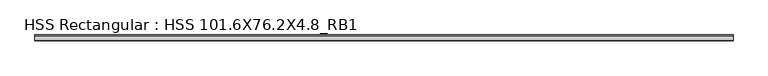
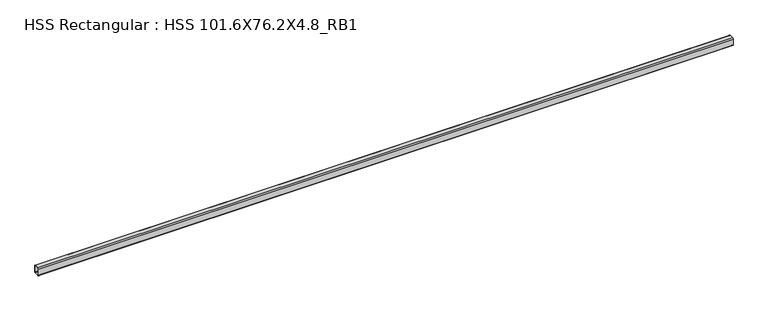
"""IFC4 building model written with IfcOpenShell, lengths in millimetres: beam geometry, HSS Rectangular : HSS 101.6X76.2X4.8_RB1."""

from ifc_helpers import new_model, si_unit, point, frame, frame_2d, origin, place, context, project, spatial, polyline, circle_curve, trimmed, segment, composite_curve, outline, extrude, source, transform, mapped, element, save


def hss_rectangular_hss_101_6x76_2x4_8_rb1_fc7daad9(model_context):
    return source(origin(), model_context, "Body", "SweptSolid", [
        extrude(outline(composite_curve([segment(polyline([(38.1, 41.275), (38.1, -41.275)]), True, "CONTINUOUS"), segment(trimmed(circle_curve(frame_2d((28.575, -41.275)), 9.525), [point((38.1, -41.275))], [point((28.575, -50.8))], False, "CARTESIAN"), True, "CONTINUOUS"), segment(polyline([(28.575, -50.8), (-28.575, -50.8)]), True, "CONTINUOUS"), segment(trimmed(circle_curve(frame_2d((-28.575, -41.275)), 9.525), [point((-28.575, -50.8))], [point((-38.1, -41.275))], False, "CARTESIAN"), True, "CONTINUOUS"), segment(polyline([(-38.1, -41.275), (-38.1, 41.275)]), True, "CONTINUOUS"), segment(trimmed(circle_curve(frame_2d((-28.575, 41.275)), 9.525), [point((-38.1, 41.275))], [point((-28.575, 50.8))], False, "CARTESIAN"), True, "CONTINUOUS"), segment(polyline([(-28.575, 50.8), (28.575, 50.8)]), True, "CONTINUOUS"), segment(trimmed(circle_curve(frame_2d((28.575, 41.275)), 9.525), [point((28.575, 50.8))], [point((38.1, 41.275))], False, "CARTESIAN"), True, "CONTINUOUS")], self_intersect=False), holes=[composite_curve([segment(trimmed(circle_curve(frame_2d((-28.575, 41.275)), 4.7625), [point((-28.575, 46.0375))], [point((-33.3375, 41.275))], True, "CARTESIAN"), True, "CONTINUOUS"), segment(polyline([(-33.3375, 41.275), (-33.3375, -41.275)]), True, "CONTINUOUS"), segment(trimmed(circle_curve(frame_2d((-28.575, -41.275)), 4.7625), [point((-33.3375, -41.275))], [point((-28.575, -46.0375))], True, "CARTESIAN"), True, "CONTINUOUS"), segment(polyline([(-28.575, -46.0375), (28.575, -46.0375)]), True, "CONTINUOUS"), segment(trimmed(circle_curve(frame_2d((28.575, -41.275)), 4.7625), [point((28.575, -46.0375))], [point((33.3375, -41.275))], True, "CARTESIAN"), True, "CONTINUOUS"), segment(polyline([(33.3375, -41.275), (33.3375, 41.275)]), True, "CONTINUOUS"), segment(trimmed(circle_curve(frame_2d((28.575, 41.275)), 4.7625), [point((33.3375, 41.275))], [point((28.575, 46.0375))], True, "CARTESIAN"), True, "CONTINUOUS"), segment(polyline([(28.575, 46.0375), (-28.575, 46.0375)]), True, "CONTINUOUS")], self_intersect=False)]), frame((-10479.1415, 0.0, 0.0), z_axis=(1.0, 0.0, 0.0), x_axis=(0.0, 1.0, 0.0)), (0.0, 0.0, 1.0), 8925.1564745),
    ])


if __name__ == "__main__":
    model = new_model("IFC4")
    model_context = context("Model", 3, world=origin())
    ifc_project = project(units=[si_unit("LENGTHUNIT", "METRE", prefix="MILLI")], contexts=[model_context])
    site = spatial("IfcSite", under=ifc_project)
    building = spatial("IfcBuilding", under=site)
    placement = place(None, origin())
    hss_rectangular_hss_101_6x76_2x4_8_rb1_shape = hss_rectangular_hss_101_6x76_2x4_8_rb1_fc7daad9(model_context)
    element("IfcBeam", 1, ObjectType="HSS Rectangular : HSS 101.6X76.2X4.8_RB1", at=placement, inside=building, context=model_context, shape_type="MappedRepresentation", body=[
        mapped(hss_rectangular_hss_101_6x76_2x4_8_rb1_shape, transform((0.0, 0.0, 0.0), x_axis=(1.0, 0.0, 0.0), y_axis=(0.0, 1.0, 0.0), z_axis=(0.0, 0.0, 1.0))),
    ])
    save(model, "model.ifc")

# Revit data of these elements
# Type "HSS Rectangular : HSS 101.6X76.2X4.8_RB1"
#   Section Name Key = "HSS 4X3X3/16"
#   Assembly Code = "B10"
#   Width = 7.62 cm
#   Wall Nominal Thickness = 0.4763 cm
#   Wall Design Thickness = 0.442 cm
#   Torsional Moment of Inertia = 260.561 cm⁴
#   Torsional Modulus = 61.2876 cm³
#   Section Area = 14.4516 cm²
#   Plastic Modulus weak axis = 40.3122 cm³
#   Plastic Modulus strong axis = 49.1612 cm³
#   Perimeter = 0.881482 m²/m
#   Outer Fillet = 0.9525 cm
#   Nominal Weight = 12.1285 kgf/m
#   Moment of Inertia weak axis = 131.529 cm⁴
#   Moment of Inertia strong axis = 205.202 cm⁴
#   Inner Fillet = 0.4763 cm
#   Height = 10.16 cm
#   Elastic Modulus weak axis = 34.4128 cm³
#   Elastic Modulus strong axis = 40.476 cm³
#   Centroid Vertical = 5.08 cm
#   Centroid Horizontal = 3.81 cm
#   Length [instance default] = 1524 mm
#   Structural Material [instance default] = Steel ASTM A500, Grade B, Rectangular and Square
#   Principal Axes Angle = 0
# Element 1 (IfcBeam, "HSS Rectangular : HSS 101.6X76.2X4.8_RB1")
#   Structural Material = Steel ASTM A992
#   Materials on its faces: "Steel ASTM A992"
# Materials
#   "Steel ASTM A500, Grade B, Rectangular and Square": class "Metal", colour RGB 199 199 199, transparency 0, Description = "Carbon steel", Cost = 0
#   "Steel ASTM A992": class "Metal", colour RGB 199 199 199, transparency 0, Description = "Structural steel 50ksi", Cost = 0
